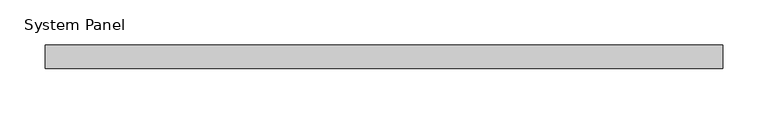
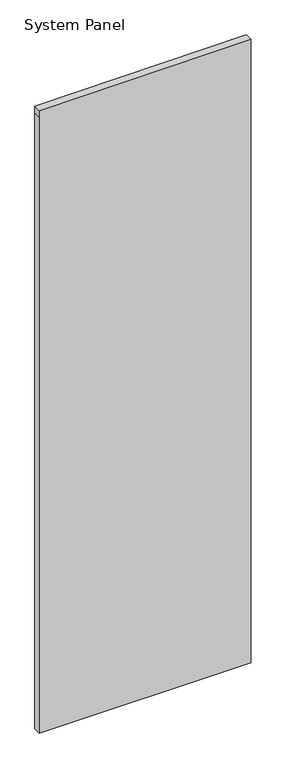
"""IFC4 building model written with IfcOpenShell, lengths in millimetres: plate geometry, System Panel : TEMPERED INSULATED GLAZING (CARDINAL GLASS LoĒ²-240."""

from ifc_helpers import new_model, si_unit, frame, origin, place, context, project, spatial, polyline, outline, extrude, source, transform, mapped, element, save


def system_panel_4a82407e(model_context):
    return source(origin(), model_context, "Body", "SweptSolid", [
        extrude(outline(polyline([(0.0, -372.4119325), (0.0, 372.4119325), (2287.5080968, 372.4119325), (2316.5806204, 372.4119325), (2311.7888098, -372.4119325), (2287.5080968, -372.4119325), (0.0, -372.4119325)])), frame((0.0, -31.75, 0.0), z_axis=(0.0, 1.0, 0.0), x_axis=(0.0, 0.0, 1.0)), (0.0, 0.0, 1.0), 25.4),
    ])


if __name__ == "__main__":
    model = new_model("IFC4")
    model_context = context("Model", 3, world=origin())
    ifc_project = project(units=[si_unit("LENGTHUNIT", "METRE", prefix="MILLI")], contexts=[model_context])
    site = spatial("IfcSite", under=ifc_project)
    building = spatial("IfcBuilding", under=site)
    placement = place(None, origin())
    system_panel_shape = system_panel_4a82407e(model_context)
    element("IfcPlate", 1, ObjectType="System Panel : TEMPERED INSULATED GLAZING (CARDINAL GLASS LoĒ²-240", at=placement, inside=building, context=model_context, shape_type="MappedRepresentation", body=[
        mapped(system_panel_shape, transform((0.0, 0.0, 0.0), x_axis=(1.0, 0.0, 0.0), y_axis=(0.0, 1.0, 0.0), z_axis=(0.0, 0.0, 1.0))),
    ])
    save(model, "model.ifc")

# Revit data of these elements
# Type "System Panel : TEMPERED INSULATED GLAZING (CARDINAL GLASS LoĒ²-240"
#   Construction Type Id = "opn-s72"
#   Analytic Construction = "Double glazing - 1/4 in thick - low-E/clear (e = 0.1) glass"
#   Visual Light Transmittance = 0.72
#   Solar Heat Gain Coefficient = 0.6
#   Heat Transfer Coefficient (U) = 1.9873 W/(m²·K)
#   Transparency_Hack = 70
# Element 1 (IfcPlate, "System Panel : TEMPERED INSULATED GLAZING (CARDINAL GLASS LoĒ²-240")
#   Materials on its faces: "TEMPERED INSULATED GLAZING (CARDINAL GLASS LoĒ²-240\nOR EQUIVALENT)"
# Materials
#   "TEMPERED INSULATED GLAZING (CARDINAL GLASS LoĒ²-240\nOR EQUIVALENT)": class "Glass", colour RGB 196 205 210, transparency 0.85, Description = "Soda Lime Glass", Cost = 0
